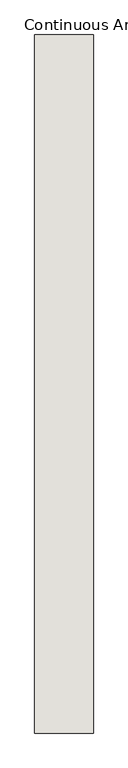
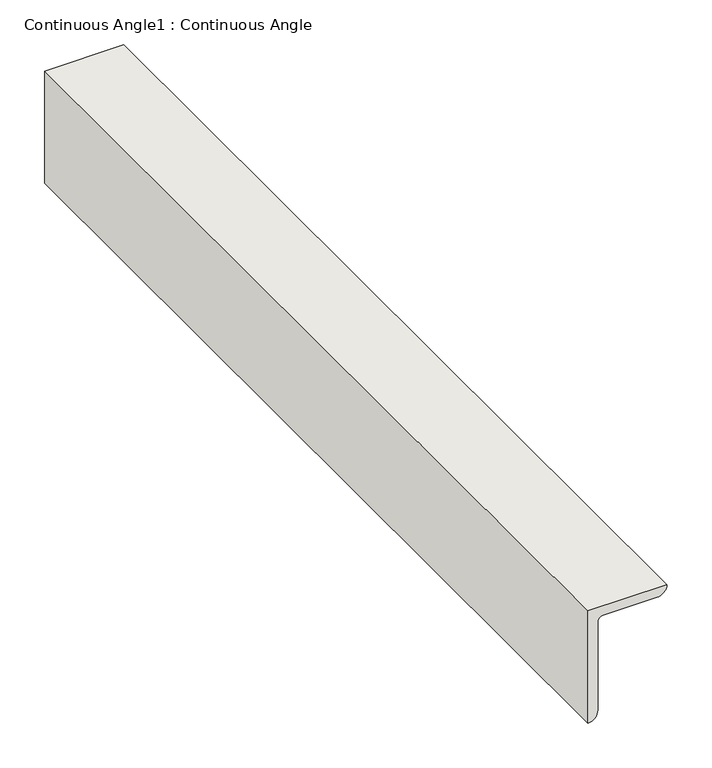
"""IFC4 building model written with IfcOpenShell, lengths in millimetres: wall geometry, Continuous Angle1 : Continuous Angle."""

from ifc_helpers import new_model, si_unit, point, frame, frame_2d, origin, place, context, project, spatial, polyline, circle_curve, trimmed, segment, composite_curve, outline, extrude, source, transform, mapped, element, save


def continuous_angle1_continuous_angle_a604bd87(model_context):
    return source(origin(), model_context, "Body", "SweptSolid", [
        extrude(outline(composite_curve([segment(polyline([(2235.2, 430198.2125), (2082.8, 430198.2125)]), True, "CONTINUOUS"), segment(trimmed(circle_curve(frame_2d((2095.5, 430198.2125)), 12.7), [point((2082.8, 430198.2125))], [point((2095.5, 430210.9125))], False, "CARTESIAN"), True, "CONTINUOUS"), segment(polyline([(2095.5, 430210.9125), (2216.15, 430210.9125)]), True, "CONTINUOUS"), segment(trimmed(circle_curve(frame_2d((2216.15, 430217.2625)), 6.35), [point((2216.15, 430210.9125))], [point((2222.5, 430217.2625))], True, "CARTESIAN"), True, "CONTINUOUS"), segment(polyline([(2222.5, 430217.2625), (2222.5, 430287.1125)]), True, "CONTINUOUS"), segment(trimmed(circle_curve(frame_2d((2235.2, 430287.1125)), 12.7), [point((2222.5, 430287.1125))], [point((2235.2, 430299.8125))], False, "CARTESIAN"), True, "CONTINUOUS"), segment(polyline([(2235.2, 430299.8125), (2235.2, 430198.2125)]), True, "CONTINUOUS")], self_intersect=False)), frame((0.0, 304.8, 0.0), z_axis=(0.0, 1.0, 0.0), x_axis=(0.0, 0.0, 1.0)), (0.0, 0.0, 1.0), 1209.675),
    ])


if __name__ == "__main__":
    model = new_model("IFC4")
    model_context = context("Model", 3, world=origin())
    ifc_project = project(units=[si_unit("LENGTHUNIT", "METRE", prefix="MILLI")], contexts=[model_context])
    site = spatial("IfcSite", under=ifc_project)
    building = spatial("IfcBuilding", under=site)
    placement = place(None, origin())
    continuous_angle1_continuous_angle_shape = continuous_angle1_continuous_angle_a604bd87(model_context)
    element("IfcWall", 1, ObjectType="Continuous Angle1 : Continuous Angle", at=placement, inside=building, context=model_context, shape_type="MappedRepresentation", body=[
        mapped(continuous_angle1_continuous_angle_shape, transform((0.0, 0.0, 0.0), x_axis=(1.0, 0.0, 0.0), y_axis=(0.0, 1.0, 0.0), z_axis=(0.0, 0.0, 1.0))),
    ])
    save(model, "model.ifc")

# Revit data of these elements
# Element 1 (IfcWall, "Continuous Angle1 : Continuous Angle")
#   Materials on its faces: "L6X4X1/2 W/ 4\" SLOT IN VERT. LOG FOR KWIK BOLT CENTER IN BLOCK (1/2\" DIA. KWIK BOLT EXPANSION ANCHOR 2.25\" EMBEDMENT aT 4FT O.C.)"
# Materials
#   "L6X4X1/2 W/ 4\" SLOT IN VERT. LOG FOR KWIK BOLT CENTER IN BLOCK (1/2\" DIA. KWIK BOLT EXPANSION ANCHOR 2.25\" EMBEDMENT aT 4FT O.C.)": class "Unassigned", colour RGB 210 209 208, transparency 0, Keynote = "M05121300.02", Cost = 0
